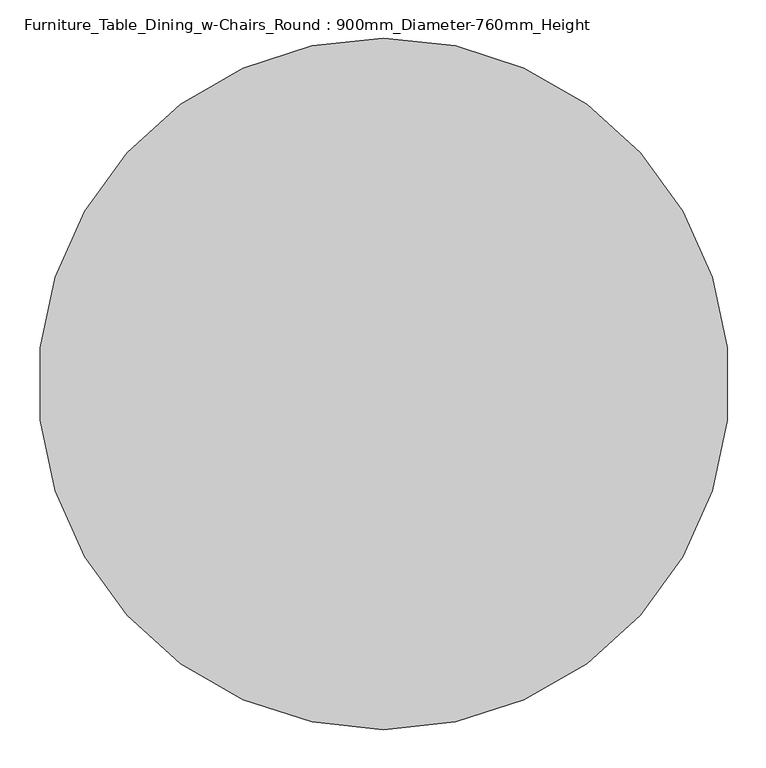
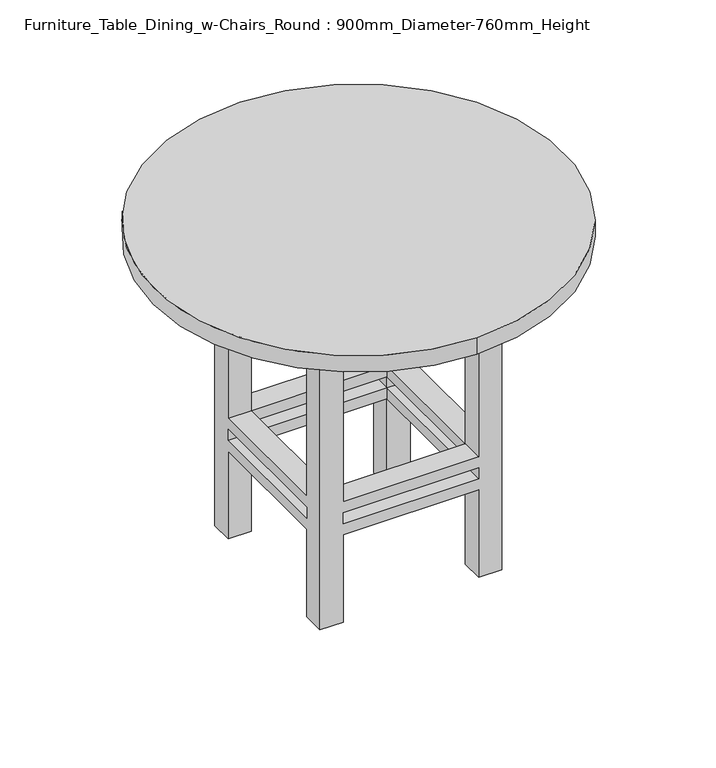
"""IFC4 building model written with IfcOpenShell, lengths in millimetres: furniture geometry, Furniture_Table_Dining_w-Chairs_Round : 900mm_Diameter-760mm_Height."""

from ifc_helpers import new_model, si_unit, point, frame, frame_2d, origin, place, context, project, spatial, polyline, circle_curve, trimmed, segment, composite_curve, outline, extrude, faceted_brep, source, transform, mapped, element, save


def furniture_table_dining_w_chairs_round_900mm_diameter_760mm_b3554e16(model_context):
    return source(origin(), model_context, "Body", "SolidModel", [
        faceted_brep([(-45.1180328, 14.7213115, 645.7), (-95.9180328, 14.7213115, 645.7), (-95.9180328, -36.0786885, 645.7), (-45.1180328, -36.0786885, 645.7), (252.4819672, 14.7213115, 645.7), (252.4819672, -36.0786885, 645.7), (303.2819672, -36.0786885, 645.7), (303.2819672, 14.7213115, 645.7), (252.4819672, -384.4786885, 645.7), (303.2819672, -384.4786885, 645.7), (303.2819672, -333.6786885, 645.7), (252.4819672, -333.6786885, 645.7), (-45.1180328, -384.4786885, 645.7), (-45.1180328, -333.6786885, 645.7), (-95.9180328, -333.6786885, 645.7), (-95.9180328, -384.4786885, 645.7), (-45.1180328, 14.7213115, 0.0), (-45.1180328, -36.0786885, 0.0), (-95.9180328, -36.0786885, 0.0), (-95.9180328, 14.7213115, 0.0), (252.4819672, 14.7213115, 0.0), (303.2819672, 14.7213115, 0.0), (303.2819672, -36.0786885, 0.0), (252.4819672, -36.0786885, 0.0), (252.4819672, -384.4786885, 0.0), (252.4819672, -333.6786885, 0.0), (303.2819672, -333.6786885, 0.0), (303.2819672, -384.4786885, 0.0), (-45.1180328, -384.4786885, 0.0), (-95.9180328, -384.4786885, 0.0), (-95.9180328, -333.6786885, 0.0), (-45.1180328, -333.6786885, 0.0), (-45.1180328, 14.7213115, 279.4), (252.4819672, 14.7213115, 279.4), (252.4819672, 14.7213115, 203.2), (-45.1180328, 14.7213115, 203.2), (252.4819672, 14.7213115, 228.6), (252.4819672, 14.7213115, 254.0), (-45.1180328, 14.7213115, 254.0), (-45.1180328, 14.7213115, 228.6), (-95.9180328, -36.0786885, 203.2), (-95.9180328, -333.6786885, 203.2), (-95.9180328, -333.6786885, 279.4), (-95.9180328, -36.0786885, 279.4), (-95.9180328, -36.0786885, 228.6), (-95.9180328, -36.0786885, 254.0), (-95.9180328, -333.6786885, 254.0), (-95.9180328, -333.6786885, 228.6), (-45.1180328, -36.0786885, 279.4), (-45.1180328, -36.0786885, 203.2), (-45.1180328, -36.0786885, 228.6), (-45.1180328, -36.0786885, 254.0), (252.4819672, -36.0786885, 279.4), (252.4819672, -36.0786885, 203.2), (252.4819672, -36.0786885, 228.6), (252.4819672, -36.0786885, 254.0), (303.2819672, -36.0786885, 279.4), (303.2819672, -36.0786885, 203.2), (303.2819672, -36.0786885, 228.6), (303.2819672, -36.0786885, 254.0), (303.2819672, -333.6786885, 279.4), (303.2819672, -333.6786885, 203.2), (303.2819672, -333.6786885, 228.6), (303.2819672, -333.6786885, 254.0), (252.4819672, -384.4786885, 279.4), (-45.1180328, -384.4786885, 279.4), (-45.1180328, -384.4786885, 203.2), (252.4819672, -384.4786885, 203.2), (-45.1180328, -384.4786885, 228.6), (-45.1180328, -384.4786885, 254.0), (252.4819672, -384.4786885, 254.0), (252.4819672, -384.4786885, 228.6), (252.4819672, -333.6786885, 279.4), (252.4819672, -333.6786885, 203.2), (252.4819672, -333.6786885, 228.6), (252.4819672, -333.6786885, 254.0), (-45.1180328, -333.6786885, 279.4), (-45.1180328, -333.6786885, 203.2), (-45.1180328, -333.6786885, 228.6), (-45.1180328, -333.6786885, 254.0)], [[[0, 1, 2, 3]], [[4, 5, 6, 7]], [[8, 9, 10, 11]], [[12, 13, 14, 15]], [[16, 17, 18, 19]], [[20, 21, 22, 23]], [[24, 25, 26, 27]], [[28, 29, 30, 31]], [[1, 0, 32, 33, 4, 7, 21, 20, 34, 35, 16, 19], [36, 37, 38, 39]], [[2, 1, 19, 18, 40, 41, 30, 29, 15, 14, 42, 43], [44, 45, 46, 47]], [[3, 2, 43, 48]], [[18, 17, 49, 40]], [[44, 50, 51, 45]], [[0, 3, 48, 32]], [[17, 16, 35, 49]], [[50, 39, 38, 51]], [[5, 4, 33, 52]], [[20, 23, 53, 34]], [[36, 54, 55, 37]], [[6, 5, 52, 56]], [[23, 22, 57, 53]], [[54, 58, 59, 55]], [[21, 7, 6, 56, 60, 10, 9, 27, 26, 61, 57, 22], [62, 63, 59, 58]], [[27, 9, 8, 64, 65, 12, 15, 29, 28, 66, 67, 24], [68, 69, 70, 71]], [[11, 10, 60, 72]], [[26, 25, 73, 61]], [[62, 74, 75, 63]], [[8, 11, 72, 64]], [[25, 24, 67, 73]], [[74, 71, 70, 75]], [[13, 12, 65, 76]], [[28, 31, 77, 66]], [[68, 78, 79, 69]], [[14, 13, 76, 42]], [[31, 30, 41, 77]], [[78, 47, 46, 79]], [[54, 74, 62, 58]], [[74, 78, 68, 71]], [[78, 50, 44, 47]], [[50, 54, 36, 39]], [[53, 49, 35, 34]], [[49, 77, 41, 40]], [[77, 73, 67, 66]], [[73, 53, 57, 61]], [[74, 54, 53, 73]], [[78, 74, 73, 77]], [[50, 78, 77, 49]], [[54, 50, 49, 53]], [[52, 72, 60, 56]], [[72, 76, 65, 64]], [[76, 48, 43, 42]], [[48, 52, 33, 32]], [[55, 51, 38, 37]], [[51, 79, 46, 45]], [[79, 75, 70, 69]], [[75, 55, 59, 63]], [[72, 52, 55, 75]], [[76, 72, 75, 79]], [[48, 76, 79, 51]], [[52, 48, 51, 55]]]),
        extrude(outline(polyline([(328.6819672, 40.1213115), (328.6819672, -409.8786885), (-121.3180328, -409.8786885), (-121.3180328, 40.1213115), (328.6819672, 40.1213115)]), holes=[polyline([(303.2819672, 14.7213115), (-95.9180328, 14.7213115), (-95.9180328, -384.4786885), (303.2819672, -384.4786885), (303.2819672, 14.7213115)])]), frame((0.0, 0.0, 645.7), z_axis=(0.0, 0.0, 1.0), x_axis=(1.0, 0.0, 0.0)), (0.0, 0.0, 1.0), 76.2),
        extrude(outline(composite_curve([segment(trimmed(circle_curve(frame_2d((103.6819672, -184.8786885)), 450.0), [point((103.6819672, -634.8786885))], [point((103.6819672, 265.1213115))], False, "CARTESIAN"), True, "CONTINUOUS"), segment(trimmed(circle_curve(frame_2d((103.6819672, -184.8786885)), 450.0), [point((103.6819672, 265.1213115))], [point((103.6819672, -634.8786885))], False, "CARTESIAN"), True, "CONTINUOUS")], self_intersect=False)), frame((0.0, 0.0, 721.9), z_axis=(0.0, 0.0, 1.0), x_axis=(1.0, 0.0, 0.0)), (0.0, 0.0, 1.0), 38.1),
    ])


if __name__ == "__main__":
    model = new_model("IFC4")
    model_context = context("Model", 3, world=origin())
    ifc_project = project(units=[si_unit("LENGTHUNIT", "METRE", prefix="MILLI")], contexts=[model_context])
    site = spatial("IfcSite", under=ifc_project)
    building = spatial("IfcBuilding", under=site)
    placement = place(None, origin())
    furniture_table_dining_w_chairs_round_900mm_diameter_760mm_shape = furniture_table_dining_w_chairs_round_900mm_diameter_760mm_b3554e16(model_context)
    element("IfcFurniture", 1, ObjectType="Furniture_Table_Dining_w-Chairs_Round : 900mm_Diameter-760mm_Height", at=placement, inside=building, context=model_context, shape_type="MappedRepresentation", body=[
        mapped(furniture_table_dining_w_chairs_round_900mm_diameter_760mm_shape, transform((0.0, 0.0, 0.0), x_axis=(1.0, 0.0, 0.0), y_axis=(0.0, 1.0, 0.0), z_axis=(0.0, 0.0, 1.0))),
    ])
    save(model, "model.ifc")

# Revit data of these elements
# Type "Furniture_Table_Dining_w-Chairs_Round : 900mm_Diameter-760mm_Height"
#   Keynote = "N"
#   Radius = 450 mm
#   Diameter = 900 mm
#   Height = 760 mm
#   Chairs = 4
#   Material Base = Wood - Pine
#   Material Top = Laminate - Linen, Matte
# Element 1 (IfcFurniture, "Furniture_Table_Dining_w-Chairs_Round : 900mm_Diameter-760mm_Height")
#   Materials on its faces: "Wood - Pine", "Laminate - Linen, Matte"
# Materials
#   "Wood - Pine": class "Wood", colour RGB 223 192 134, transparency 0
#   "Laminate - Linen, Matte": class "Miscellaneous", colour RGB 249 239 230, transparency 0
